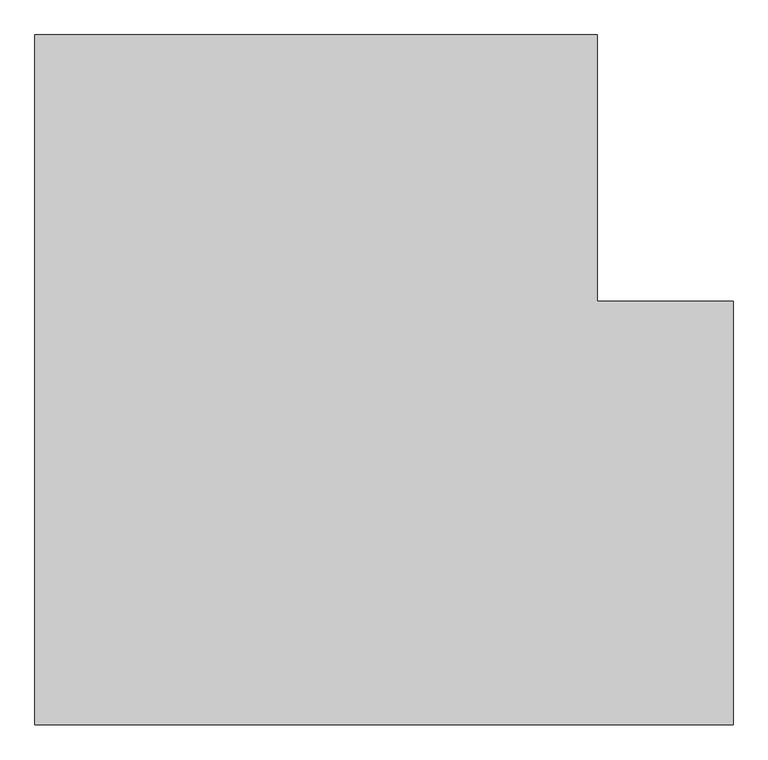
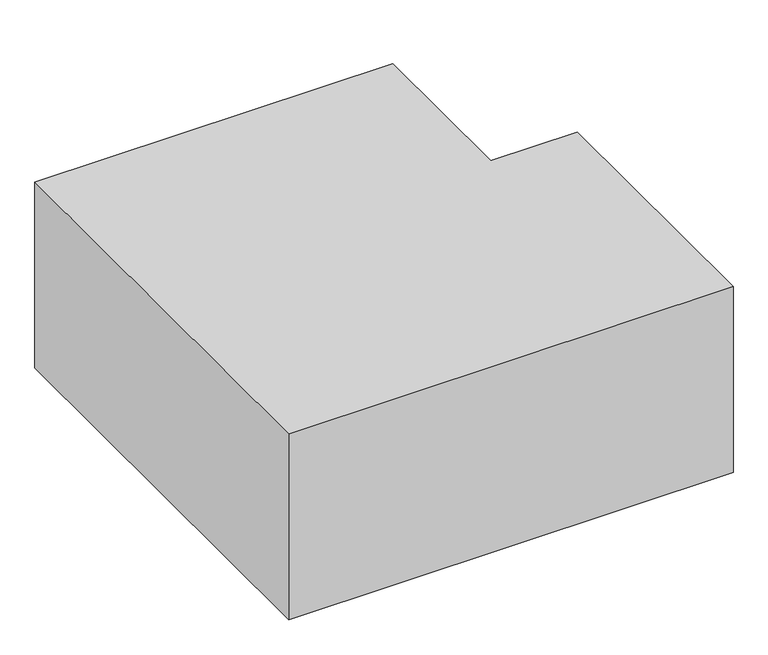
"""IFC4 building model written with IfcOpenShell, lengths in millimetres: proxy geometry, 0_3d."""

from ifc_helpers import new_model, si_unit, origin, origin_with_axes, place, context, project, spatial, polyline, outline, extrude, source, transform, mapped, element, save


def generic_models_805eeb56(model_context):
    return source(origin(), model_context, "Body", "SweptSolid", [
        extrude(outline(polyline([(5650.0, 3427.8619019), (5649.840708, 0.0), (0.0, 0.0), (0.0, 5582.8619019), (4550.0, 5582.8619019), (4550.0, 3427.8619019), (5650.0, 3427.8619019)])), origin_with_axes(), (0.0, 0.0, 1.0), 2500.0),
    ])


if __name__ == "__main__":
    model = new_model("IFC4")
    model_context = context("Model", 3, world=origin())
    ifc_project = project(units=[si_unit("LENGTHUNIT", "METRE", prefix="MILLI")], contexts=[model_context])
    site = spatial("IfcSite", under=ifc_project)
    building = spatial("IfcBuilding", under=site)
    placement = place(None, origin())
    generic_models_shape = generic_models_805eeb56(model_context)
    element("IfcBuildingElementProxy", 1, Name="0_3d", ObjectType="0_3d", at=placement, inside=building, context=model_context, shape_type="MappedRepresentation", body=[
        mapped(generic_models_shape, transform((0.0, 0.0, 0.0), x_axis=(1.0, 0.0, 0.0), y_axis=(0.0, 1.0, 0.0), z_axis=(0.0, 0.0, 1.0))),
    ])
    save(model, "model.ifc")

# Revit data of these elements
# Element 1 (IfcBuildingElementProxy, "0_3d")
#   Materials on its faces: "*1"
# Materials
#   "*1": class "Unassigned", colour RGB 175 175 175, transparency 0
